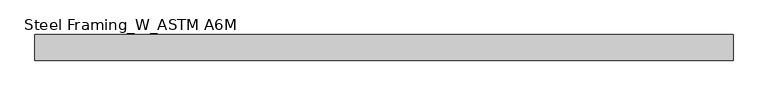
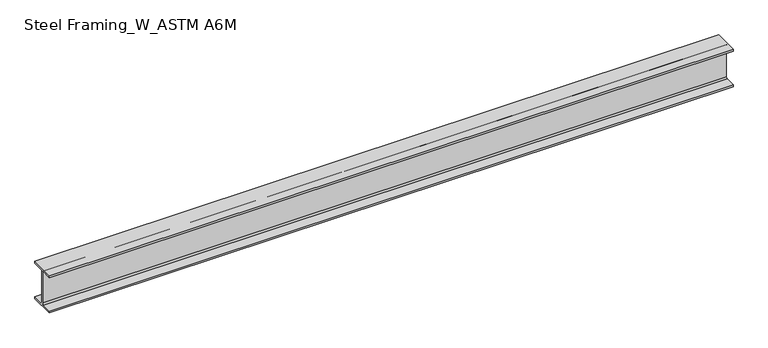
"""IFC4 building model written with IfcOpenShell, lengths in millimetres: beam geometry, Steel Framing_W_ASTM A6M : H_SB_AR_S02_W200x31.3_B6."""

from ifc_helpers import new_model, si_unit, point, frame, frame_2d, origin, place, context, project, spatial, polyline, circle_curve, trimmed, segment, composite_curve, outline, extrude, source, transform, mapped, element, save


def steel_framing_w_astm_a6m_8ca0da9a(model_context):
    return source(origin(), model_context, "Body", "SweptSolid", [
        extrude(outline(composite_curve([segment(polyline([(67.0, -94.8), (67.0, -105.0), (-67.0, -105.0), (-67.0, -94.8), (-10.775, -94.8)]), True, "CONTINUOUS"), segment(trimmed(circle_curve(frame_2d((-10.775, -87.2)), 7.6), [point((-10.775, -94.8))], [point((-3.175, -87.2))], True, "CARTESIAN"), True, "CONTINUOUS"), segment(polyline([(-3.175, -87.2), (-3.175, 87.2)]), True, "CONTINUOUS"), segment(trimmed(circle_curve(frame_2d((-10.775, 87.2)), 7.6), [point((-3.175, 87.2))], [point((-10.775, 94.8))], True, "CARTESIAN"), True, "CONTINUOUS"), segment(polyline([(-10.775, 94.8), (-67.0, 94.8), (-67.0, 105.0), (67.0, 105.0), (67.0, 94.8), (10.775, 94.8)]), True, "CONTINUOUS"), segment(trimmed(circle_curve(frame_2d((10.775, 87.2)), 7.6), [point((10.775, 94.8))], [point((3.175, 87.2))], True, "CARTESIAN"), True, "CONTINUOUS"), segment(polyline([(3.175, 87.2), (3.175, -87.2)]), True, "CONTINUOUS"), segment(trimmed(circle_curve(frame_2d((10.775, -87.2)), 7.6), [point((3.175, -87.2))], [point((10.775, -94.8))], True, "CARTESIAN"), True, "CONTINUOUS"), segment(polyline([(10.775, -94.8), (67.0, -94.8)]), True, "CONTINUOUS")], self_intersect=False)), frame((-1802.5, 0.0, 0.0), z_axis=(1.0, 0.0, 0.0), x_axis=(0.0, 1.0, 0.0)), (0.0, 0.0, 1.0), 3648.8),
    ])


if __name__ == "__main__":
    model = new_model("IFC4")
    model_context = context("Model", 3, world=origin())
    ifc_project = project(units=[si_unit("LENGTHUNIT", "METRE", prefix="MILLI")], contexts=[model_context])
    site = spatial("IfcSite", under=ifc_project)
    building = spatial("IfcBuilding", under=site)
    placement = place(None, origin())
    steel_framing_w_astm_a6m_shape = steel_framing_w_astm_a6m_8ca0da9a(model_context)
    element("IfcBeam", 1, ObjectType="Steel Framing_W_ASTM A6M : H_SB_AR_S02_W200x31.3_B6", at=placement, inside=building, context=model_context, shape_type="MappedRepresentation", body=[
        mapped(steel_framing_w_astm_a6m_shape, transform((0.0, 0.0, 0.0), x_axis=(1.0, 0.0, 0.0), y_axis=(0.0, 1.0, 0.0), z_axis=(0.0, 0.0, 1.0))),
    ])
    save(model, "model.ifc")

# Revit data of these elements
# Type "Steel Framing_W_ASTM A6M : H_SB_AR_S02_W200x31.3_B6"
#   Type Mark = "B6"
#   Section Name Key = "W8x21"
#   Width = 13.4 cm
#   Web Thickness = 0.635 cm
#   Web Fillet = 0.76 cm
#   Warping Constant = 40800.0 cm⁶
#   Torsional Moment of Inertia = 11.70 cm⁴
#   Section Area = 39.7 cm²
#   Plastic Modulus weak axis = 93.2 cm³
#   Plastic Modulus strong axis = 334.0 cm³
#   Perimeter = 0.93 m²/m
#   Nominal Weight = 31.30 kgf/m
#   Moment of Inertia weak axis = 407.00 cm⁴
#   Moment of Inertia strong axis = 3130.00 cm⁴
#   Height = 21.0 cm
#   Flange Thickness = 1.02 cm
#   Elastic Modulus weak axis = 60.8 cm³
#   Elastic Modulus strong axis = 298.0 cm³
#   Centroid Vertical = 10.5 cm
#   Centroid Horizontal = 6.7 cm
#   Length [instance default] = 1500 mm
#   Structural Material [instance default] = Steel, 45-345
#   Bolt Spacing = 0
#   Assembly Code = ""
# Element 1 (IfcBeam, "Steel Framing_W_ASTM A6M : H_SB_AR_S02_W200x31.3_B6")
#   Materials on its faces: "Steel, 45-345"
# Materials
#   "Steel, 45-345": class "Metal", colour RGB 189 187 185, transparency 0, Description = "Steel 345 MPa", Cost = 0
